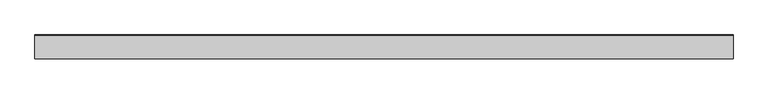
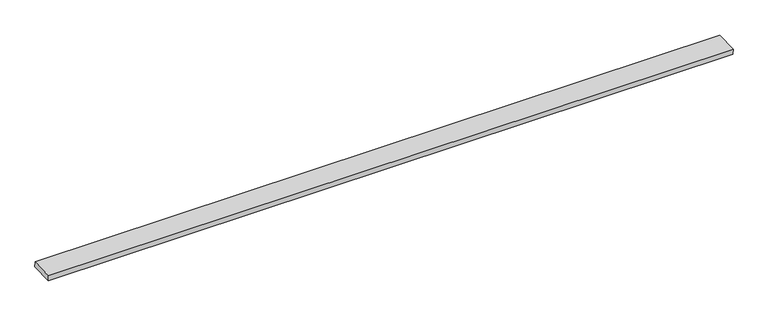
"""IFC4 building model written with IfcOpenShell, lengths in millimetres: proxy geometry, Generic Models 7:Generic Models 1:2:Generic Models 1:2 : Generic Models 7:Generic Models 1:337419:6 : Generic Models 7:Generic Models 1:2:Generic Models 1:2 : Generic Models 7:Generic Models 1:337419:306751."""

from ifc_helpers import new_model, si_unit, frame, origin, place, context, project, spatial, polyline, outline, extrude, source, transform, mapped, element, save


def generic_models_bfa17058(model_context):
    return source(origin(), model_context, "Body", "SweptSolid", [
        extrude(outline(polyline([(0.0, -164.842211), (0.0, 0.0), (4876.8, 0.0), (4876.8, -164.842211), (0.0, -164.842211)])), frame((596182.8367239, -568179.2782965, 8524.3603203), z_axis=(0.0, -0.041630544767773385, 0.9991330730900356), x_axis=(-1.0, 0.0, 0.0)), (0.0, 0.0, 1.0), 38.1),
    ])


if __name__ == "__main__":
    model = new_model("IFC4")
    model_context = context("Model", 3, world=origin())
    ifc_project = project(units=[si_unit("LENGTHUNIT", "METRE", prefix="MILLI")], contexts=[model_context])
    site = spatial("IfcSite", under=ifc_project)
    building = spatial("IfcBuilding", under=site)
    placement = place(None, origin())
    generic_models_shape = generic_models_bfa17058(model_context)
    element("IfcBuildingElementProxy", 1, Name="Generic Models 7:Generic Models 1:2:Generic Models 1:2 : Generic Models 7:Generic Models 1:337419:6 : Generic Models 7:Generic Models 1:2:Generic Models 1:2 : Generic Models 7:Generic Models 1:337419:306751", ObjectType="Generic Models 7:Generic Models 1:2:Generic Models 1:2 : Generic Models 7:Generic Models 1:337419:6 : Generic Models 7:Generic Models 1:2:Generic Models 1:2 : Generic Models 7:Generic Models 1:337419:306751", at=placement, inside=building, context=model_context, shape_type="MappedRepresentation", body=[
        mapped(generic_models_shape, transform((0.0, 0.0, 0.0), x_axis=(1.0, 0.0, 0.0), y_axis=(0.0, 1.0, 0.0), z_axis=(0.0, 0.0, 1.0))),
    ])
    save(model, "model.ifc")

# Revit data of these elements
# Type "Generic Models 7:Generic Models 1:2:Generic Models 1:2 : Generic Models 7:Generic Models 1:337419:6 : Generic Models 7:Generic Models 1:2:Generic Models 1:2 : Generic Models 7:Generic Models 1:337419:306751"
#   NameOverride = "Generic Models 7:Generic Models 1:2:Generic Models 1:2 : Generic Models 7:Generic Models 1:337419:306751"
#   ObjectTypeOverride = "Generic Models 1:2 : Generic Models 7:Generic Models 1:337419"
#   Reference = "Generic Models 1"
#   Tag = "306751"
# Element 1 (IfcBuildingElementProxy, "Generic Models 7:Generic Models 1:2:Generic Models 1:2 : Generic Models 7:Generic Models 1:337419:6 : Generic Models 7:Generic Models 1:2:Generic Models 1:2 : Generic Models 7:Generic Models 1:337419:306751")
#   Materials on its faces: "FIRE RETARDTANT WOOD BLOCKING - SIZE AS NEC."
# Materials
#   "FIRE RETARDTANT WOOD BLOCKING - SIZE AS NEC.": class "Wood", colour RGB 144 113 62, transparency 0, Description = "Pinus Echinata", Cost = 0
